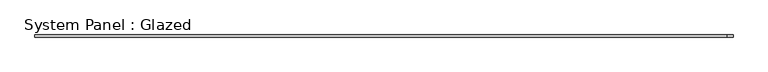
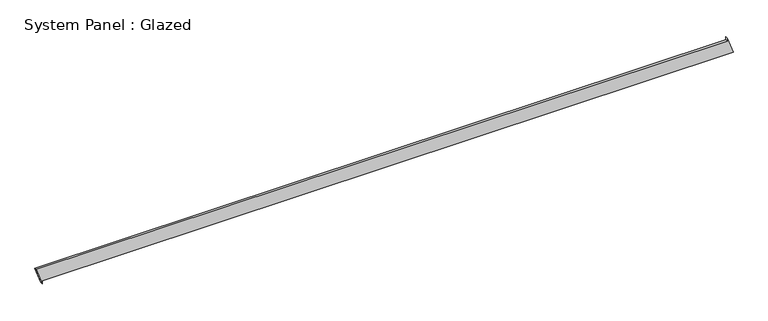
"""IFC4 building model written with IfcOpenShell, lengths in millimetres: plate geometry, System Panel : Glazed."""

from ifc_helpers import new_model, si_unit, frame, origin, place, context, project, spatial, polyline, outline, extrude, source, transform, mapped, element, save


def system_panel_glazed_126292fd(model_context):
    return source(origin(), model_context, "Body", "SweptSolid", [
        extrude(outline(polyline([(0.0, -3959.2825517), (35.3553391, -3959.2825517), (35.3553391, 4028.0914575), (234.6663814, 3959.2041333), (199.3110424, 3959.2039893), (199.3435652, -4028.0914575), (0.0, -3959.2825517)])), frame((0.0, -49.5, 0.0), z_axis=(0.0, 1.0, 0.0), x_axis=(0.0, 0.0, 1.0)), (0.0, 0.0, 1.0), 25.0),
    ])


if __name__ == "__main__":
    model = new_model("IFC4")
    model_context = context("Model", 3, world=origin())
    ifc_project = project(units=[si_unit("LENGTHUNIT", "METRE", prefix="MILLI")], contexts=[model_context])
    site = spatial("IfcSite", under=ifc_project)
    building = spatial("IfcBuilding", under=site)
    placement = place(None, origin())
    system_panel_glazed_shape = system_panel_glazed_126292fd(model_context)
    element("IfcPlate", 1, ObjectType="System Panel : Glazed", at=placement, inside=building, context=model_context, shape_type="MappedRepresentation", body=[
        mapped(system_panel_glazed_shape, transform((0.0, 0.0, 0.0), x_axis=(1.0, 0.0, 0.0), y_axis=(0.0, 1.0, 0.0), z_axis=(0.0, 0.0, 1.0))),
    ])
    save(model, "model.ifc")

# Revit data of these elements
# Element 1 (IfcPlate, "System Panel : Glazed")
#   Materials on its faces: "Glass"
# Materials
#   "Glass": class "Glass", colour RGB 218 227 224, transparency 0.85, Description = "Soda Lime Glass", Cost = 0
